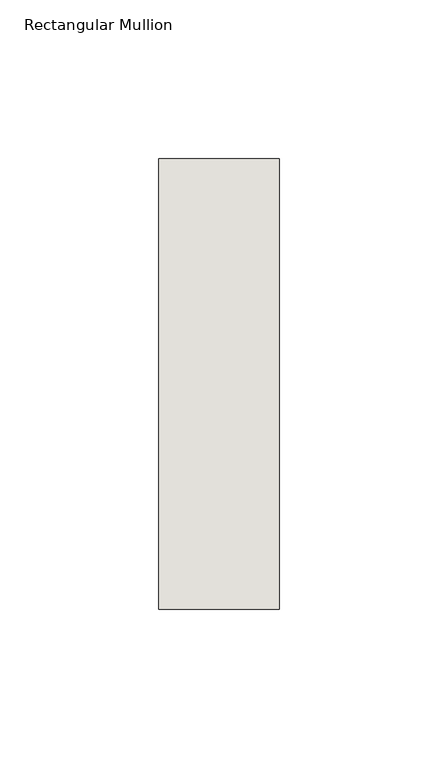
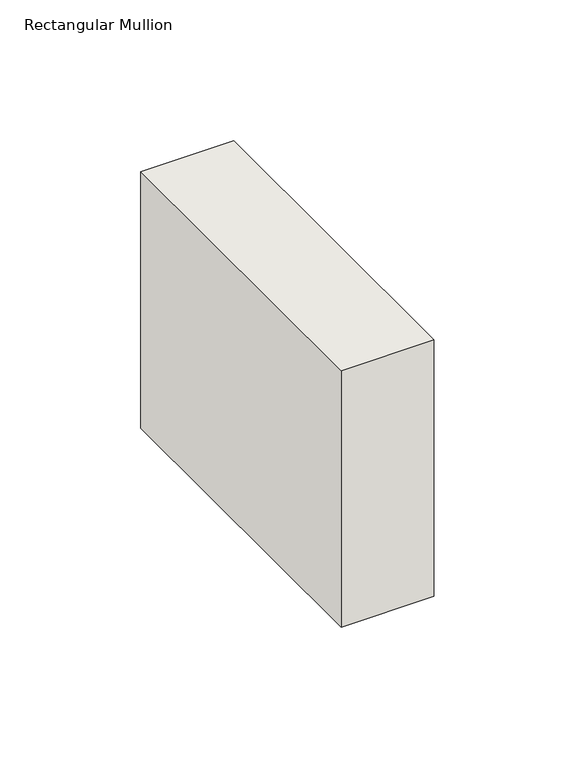
"""IFC4 building model written with IfcOpenShell, lengths in millimetres: wall geometry, Rectangular Mullion : NLRS_21_CWM_hsb-regel 38x142_gen_rsf."""

from ifc_helpers import new_model, si_unit, frame, origin, place, context, project, spatial, polyline, outline, extrude, source, transform, mapped, element, save


def rectangular_mullion_8b5cfd33(model_context):
    return source(origin(), model_context, "Body", "SweptSolid", [
        extrude(outline(polyline([(0.0, -71.0), (-38.0, -71.0), (-38.0, 71.0), (0.0, 71.0), (0.0, -71.0)])), frame((0.0, 0.0, -111.0), z_axis=(0.0, 0.0, 1.0), x_axis=(1.0, 0.0, 0.0)), (0.0, 0.0, 1.0), 111.0),
    ])


if __name__ == "__main__":
    model = new_model("IFC4")
    model_context = context("Model", 3, world=origin())
    ifc_project = project(units=[si_unit("LENGTHUNIT", "METRE", prefix="MILLI")], contexts=[model_context])
    site = spatial("IfcSite", under=ifc_project)
    building = spatial("IfcBuilding", under=site)
    placement = place(None, origin())
    rectangular_mullion_shape = rectangular_mullion_8b5cfd33(model_context)
    element("IfcWall", 1, ObjectType="Rectangular Mullion : NLRS_21_CWM_hsb-regel 38x142_gen_rsf", at=placement, inside=building, context=model_context, shape_type="MappedRepresentation", body=[
        mapped(rectangular_mullion_shape, transform((0.0, 0.0, 0.0), x_axis=(1.0, 0.0, 0.0), y_axis=(0.0, 1.0, 0.0), z_axis=(0.0, 0.0, 1.0))),
    ])
    save(model, "model.ifc")

# Revit data of these elements
# Type "Rectangular Mullion : NLRS_21_CWM_hsb-regel 38x142_gen_rsf"
#   Type IfcGUID = "07M7mRoiH1CR8m_RSKIwpF"
#   Assembly Code = "21.10"
#   IfcExportAs = "IfcWall"
#   built-in parameter 1007322 = 0.465879 (stored number, unit not read)
#   built-in parameter 1007321 = 0.062336 (stored number, unit not read)
#   built-in parameter 1007320 = 0.062336 (stored number, unit not read)
# Element 1 (IfcWall, "Rectangular Mullion : NLRS_21_CWM_hsb-regel 38x142_gen_rsf")
#   Materials on its faces: "NLRS_i2_hout naaldhout vuren_gen_rsf"
# Materials
#   "NLRS_i2_hout naaldhout vuren_gen_rsf": class "I - Hout", colour RGB 234 199 147, transparency 0, Keynote = "i2", Manufacturer = "Revit Standards Foundation", URL = "www.revitstandards.org", Description = "hout vuren", Cost = 0
